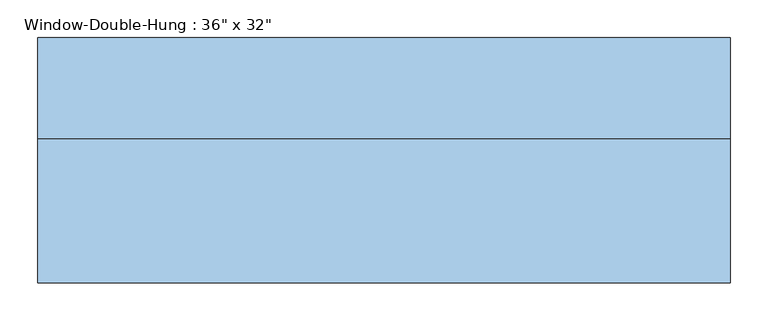
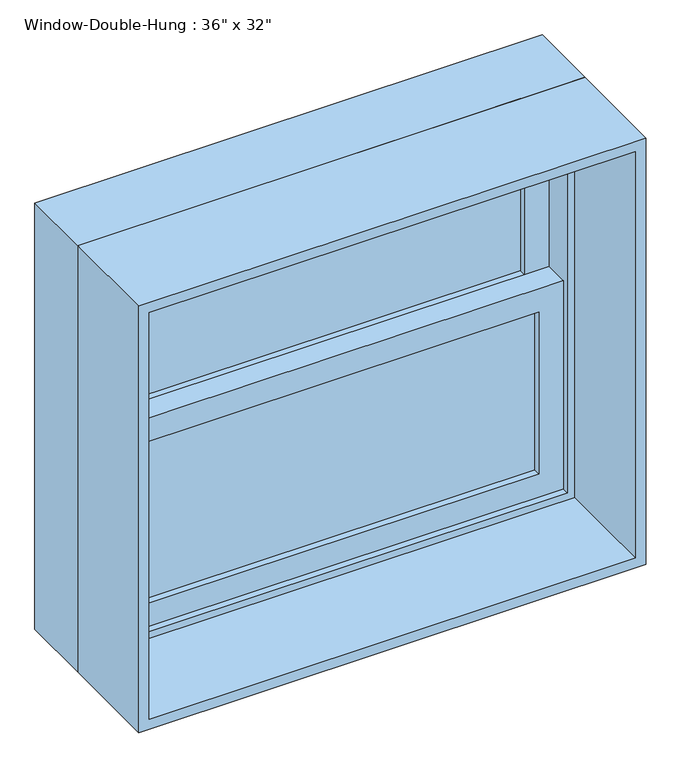
"""IFC4 building model written with IfcOpenShell, lengths in millimetres: window geometry."""

from ifc_helpers import new_model, si_unit, frame, origin, place, context, project, spatial, polyline, outline, extrude, source, transform, mapped, element, save


def window_e3cc3ff6(model_context):
    return source(origin(), model_context, "Body", "SweptSolid", [
        extrude(outline(polyline([(381.0, 82.55), (381.0, 76.2), (-381.0, 76.2), (-381.0, 82.55), (381.0, 82.55)])), frame((0.0, 0.0, 990.6), z_axis=(0.0, 0.0, 1.0), x_axis=(1.0, 0.0, 0.0)), (0.0, 0.0, 1.0), 307.975),
        extrude(outline(polyline([(-381.0, 69.85), (381.0, 69.85), (381.0, 63.5), (-381.0, 63.5), (-381.0, 69.85)])), frame((0.0, 0.0, 990.6), z_axis=(0.0, 0.0, 1.0), x_axis=(1.0, 0.0, 0.0)), (0.0, 0.0, 1.0), 307.975),
        extrude(outline(polyline([(381.0, 127.0), (381.0, 120.65), (-381.0, 120.65), (-381.0, 127.0), (381.0, 127.0)])), frame((0.0, 0.0, 1343.025), z_axis=(0.0, 0.0, 1.0), x_axis=(1.0, 0.0, 0.0)), (0.0, 0.0, 1.0), 307.975),
        extrude(outline(polyline([(-381.0, 114.3), (381.0, 114.3), (381.0, 107.95), (-381.0, 107.95), (-381.0, 114.3)])), frame((0.0, 0.0, 1343.025), z_axis=(0.0, 0.0, 1.0), x_axis=(1.0, 0.0, 0.0)), (0.0, 0.0, 1.0), 307.975),
        extrude(outline(polyline([(1343.025, -425.45), (946.15, -425.45), (946.15, 425.45), (1343.025, 425.45), (1343.025, -425.45)]), holes=[polyline([(1298.575, 381.0), (990.6, 381.0), (990.6, -381.0), (1298.575, -381.0), (1298.575, 381.0)])]), frame((0.0, 50.8, 0.0), z_axis=(0.0, 1.0, 0.0), x_axis=(0.0, 0.0, 1.0)), (0.0, 0.0, 1.0), 44.45),
        extrude(outline(polyline([(1695.45, -425.45), (1298.575, -425.45), (1298.575, 425.45), (1695.45, 425.45), (1695.45, -425.45)]), holes=[polyline([(1651.0, 381.0), (1343.025, 381.0), (1343.025, -381.0), (1651.0, -381.0), (1651.0, 381.0)])]), frame((0.0, 95.25, 0.0), z_axis=(0.0, 1.0, 0.0), x_axis=(0.0, 0.0, 1.0)), (0.0, 0.0, 1.0), 44.45),
        extrude(outline(polyline([(1727.2, -457.2), (914.4, -457.2), (914.4, 457.2), (1727.2, 457.2), (1727.2, -457.2)]), holes=[polyline([(1695.45, 425.45), (946.15, 425.45), (946.15, -425.45), (1695.45, -425.45), (1695.45, 425.45)])]), frame((0.0, 38.1, 0.0), z_axis=(0.0, 1.0, 0.0), x_axis=(0.0, 0.0, 1.0)), (0.0, 0.0, 1.0), 133.35),
        extrude(outline(polyline([(1727.2, 457.2), (1727.2, -457.2), (914.4, -457.2), (914.4, 457.2), (1727.2, 457.2)]), holes=[polyline([(1708.15, 438.15), (933.45, 438.15), (933.45, -438.15), (1708.15, -438.15), (1708.15, 438.15)])]), frame((0.0, -152.4, 0.0), z_axis=(0.0, 1.0, 0.0), x_axis=(0.0, 0.0, 1.0)), (0.0, 0.0, 1.0), 190.5),
    ])


if __name__ == "__main__":
    model = new_model("IFC4")
    model_context = context("Model", 3, world=origin())
    ifc_project = project(units=[si_unit("LENGTHUNIT", "METRE", prefix="MILLI")], contexts=[model_context])
    site = spatial("IfcSite", under=ifc_project)
    building = spatial("IfcBuilding", under=site)
    placement = place(None, origin())
    window_shape = window_e3cc3ff6(model_context)
    element("IfcWindow", 1, ObjectType="Window-Double-Hung : 36\" x 32\"", at=placement, inside=building, context=model_context, shape_type="MappedRepresentation", body=[
        mapped(window_shape, transform((0.0, 0.0, 0.0), x_axis=(1.0, 0.0, 0.0), y_axis=(0.0, 1.0, 0.0), z_axis=(0.0, 0.0, 1.0))),
    ])
    save(model, "model.ifc")

# Revit data of these elements
# Type "Window-Double-Hung : 36\" x 32\""
#   Type Mark = "19"
#   Fire Rating = "0.5h"
#   Construction Type Id = "DG-DR"
#   Assembly Code = "B2020100"
#   Analytic Construction = "Double glazing - domestic"
#   Wall Thickness [instance default] = 0' - 6"
#   Window Inset [instance default] = 0' - 0"
#   Visual Light Transmittance = 0.81
#   Thermal Resistance (R) = 1.8146 (h·ft²·°F)/BTU
#   Solar Heat Gain Coefficient = 0.76
#   Muntin Width = 2' - 6"
#   Muntin Height = 1' - 0 1/8"
#   Interior Wall Closure [instance default] = 0' - 1 1/2"
#   Rough Width = 3' - 0 1/2"
#   Rough Height = 2' - 8 1/2"
#   Frame Extension [instance default] = 0' - 1 1/4"
#   Exterior Wall Closure [instance default] = 0' - 0 1/2"
#   Extension Jamb [instance default] = 0' - 1 1/2"
#   Heat Transfer Coefficient (U) = 0.5511 BTU/(h·ft²·°F)
#   Height = 2' - 8"
#   Width = 3' - 0"
#   Top Muntin Visibility = yes
#   Indicator Visibility [instance default] = yes
#   Extension Jamb Visibility [instance default] = yes
#   Interior Trim Visibility [instance default] = yes
#   Exterior Trim Visibility [instance default] = yes
#   Define Thermal Properties by = 1
#   Bottom Muntin Visibility = yes
#   Muntin Pattern = Muntin Pattern_2x2 : Muntin Pattern_2x2
#   Interior Trim Material = Wood - Stained
#   Interior Trim = Trim-Window-Interior-Flat : Picture Frame
#   Exterior Trim Material = Clad - White
#   Exterior Trim = Trim-Window-Exterior-Flat : with Sill
#   Glass Panel Material = Glass
#   Exterior Frame Material = Clad - White
#   Interior Frame Material = Wood - Stained
#   Wall Closure = (empty or 0)
# Element 1 (IfcWindow, "Window-Double-Hung : 36\" x 32\"")
#   Wall Thickness = 1' - 0"
#   Extension Jamb = 0' - 7 1/2"
#   Materials on its faces: "Wood - Stained", "Glass", "Clad - White"
# Materials
#   "Wood - Stained": class "Wood", colour RGB 224 178 126, transparency 0, Cost = 0
#   "Clad - White": class "Wood", colour RGB 242 242 238, transparency 0, Cost = 0
#   "Glass": class "Glass", colour RGB 0 128 192, transparency 0.75, Description = "Soda Lime Glass", Cost = 0
